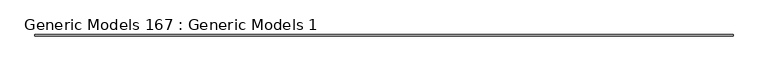
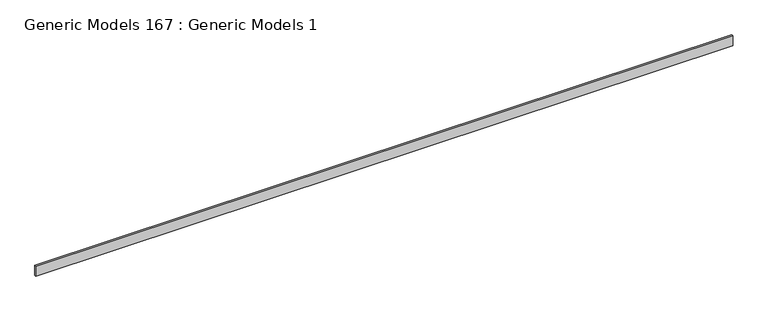
"""IFC4 building model written with IfcOpenShell, lengths in millimetres: proxy geometry, Generic Models 167 : Generic Models 1."""

from ifc_helpers import new_model, si_unit, frame, origin, place, context, project, spatial, polyline, outline, extrude, source, transform, mapped, element, save


def generic_models_167_generic_models_1_7743eff9(model_context):
    return source(origin(), model_context, "Body", "SweptSolid", [
        extrude(outline(polyline([(-10459.9421316, -7052.2480338), (-10459.9421316, -7014.1480338), (8590.0578684, -7014.1480338), (8590.0578684, -7052.2480338), (-10459.9421316, -7052.2480338)])), frame((0.0, 0.0, 126466.346), z_axis=(0.0, 0.0, 1.0), x_axis=(1.0, 0.0, 0.0)), (0.0, 0.0, 1.0), 285.75),
    ])


if __name__ == "__main__":
    model = new_model("IFC4")
    model_context = context("Model", 3, world=origin())
    ifc_project = project(units=[si_unit("LENGTHUNIT", "METRE", prefix="MILLI")], contexts=[model_context])
    site = spatial("IfcSite", under=ifc_project)
    building = spatial("IfcBuilding", under=site)
    placement = place(None, origin())
    generic_models_167_generic_models_1_shape = generic_models_167_generic_models_1_7743eff9(model_context)
    element("IfcBuildingElementProxy", 1, Name="Generic Models 167 : Generic Models 1", ObjectType="Generic Models 167 : Generic Models 1", at=placement, inside=building, context=model_context, shape_type="MappedRepresentation", body=[
        mapped(generic_models_167_generic_models_1_shape, transform((0.0, 0.0, 0.0), x_axis=(1.0, 0.0, 0.0), y_axis=(0.0, 1.0, 0.0), z_axis=(0.0, 0.0, 1.0))),
    ])
    save(model, "model.ifc")

# Revit data of these elements
# Element 1 (IfcBuildingElementProxy, "Generic Models 167 : Generic Models 1")
#   Materials on its faces: "_STRUCTURAL MEMBER (SEE STRUCT. DWGS)"
# Materials
#   "_STRUCTURAL MEMBER (SEE STRUCT. DWGS)": class "Generic", colour RGB 209 182 141, transparency 0, Cost = 0
